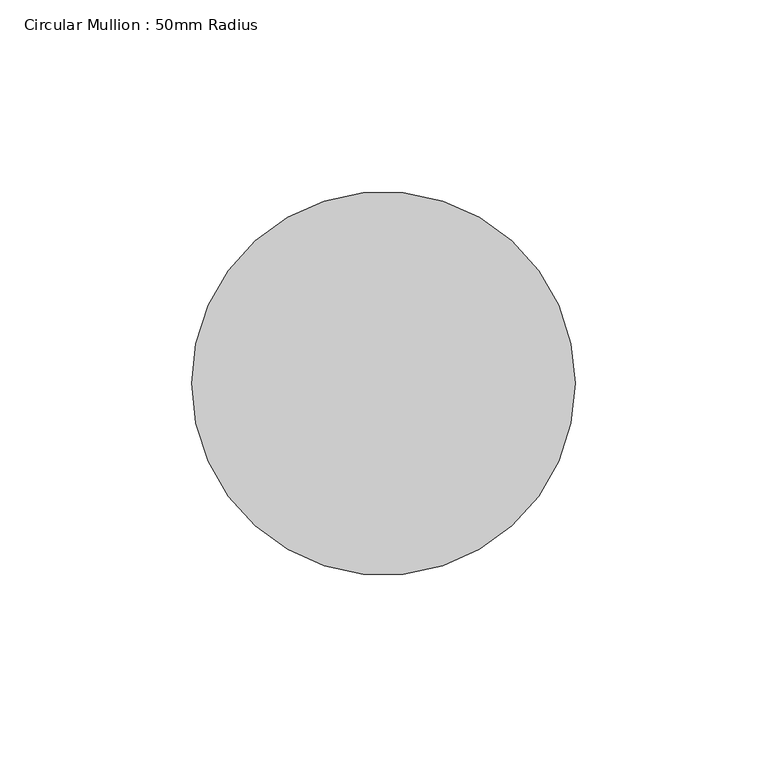
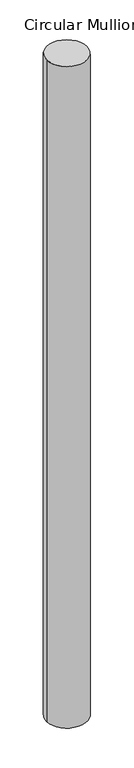
"""IFC4 building model written with IfcOpenShell, lengths in millimetres: member geometry, Circular Mullion : 50mm Radius."""

from ifc_helpers import new_model, si_unit, point, frame, origin, origin_2d, place, context, project, spatial, circle_curve, trimmed, segment, composite_curve, outline, extrude, source, transform, mapped, element, save


def circular_mullion_50mm_radius_a4d1b6b9(model_context):
    return source(origin(), model_context, "Body", "SweptSolid", [
        extrude(outline(composite_curve([segment(trimmed(circle_curve(origin_2d(), 50.0), [point((50.0, 0.0))], [point((-50.0, 0.0))], False, "CARTESIAN"), True, "CONTINUOUS"), segment(trimmed(circle_curve(origin_2d(), 50.0), [point((-50.0, 0.0))], [point((50.0, 0.0))], False, "CARTESIAN"), True, "CONTINUOUS")], self_intersect=False)), frame((0.0, 0.0, -1731.8314335), z_axis=(0.0, 0.0, 1.0), x_axis=(1.0, 0.0, 0.0)), (0.0, 0.0, 1.0), 1731.8314335),
    ])


if __name__ == "__main__":
    model = new_model("IFC4")
    model_context = context("Model", 3, world=origin())
    ifc_project = project(units=[si_unit("LENGTHUNIT", "METRE", prefix="MILLI")], contexts=[model_context])
    site = spatial("IfcSite", under=ifc_project)
    building = spatial("IfcBuilding", under=site)
    placement = place(None, origin())
    circular_mullion_50mm_radius_shape = circular_mullion_50mm_radius_a4d1b6b9(model_context)
    element("IfcMember", 1, ObjectType="Circular Mullion : 50mm Radius", at=placement, inside=building, context=model_context, shape_type="MappedRepresentation", body=[
        mapped(circular_mullion_50mm_radius_shape, transform((0.0, 0.0, 0.0), x_axis=(1.0, 0.0, 0.0), y_axis=(0.0, 1.0, 0.0), z_axis=(0.0, 0.0, 1.0))),
    ])
    save(model, "model.ifc")

# Revit data of these elements
# Type "Circular Mullion : 50mm Radius"
#   built-in parameter 1007350 = 0.164042 (stored number, unit not read)
# Element 1 (IfcMember, "Circular Mullion : 50mm Radius")
#   Materials on its faces: "Aluminium"
# Materials
#   "Aluminium": class "Metal", colour RGB 247 247 247, transparency 0, Description = "Aluminium 6061", Cost = 0
